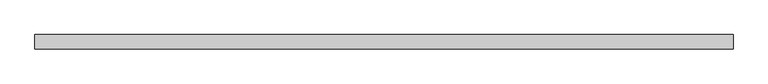
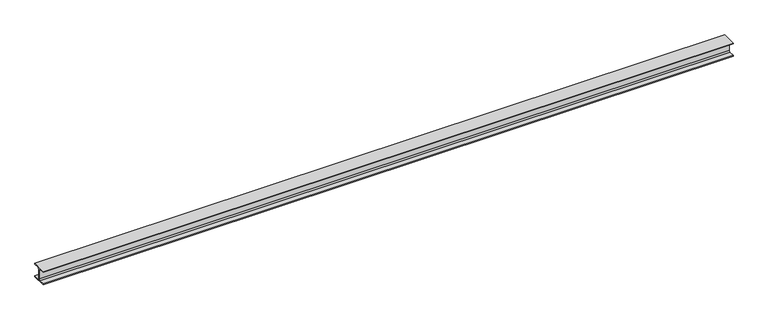
"""IFC4 building model written with IfcOpenShell, lengths in millimetres: beam geometry, NLRS_28_SF_LIB_stalen ligger HEB-AV-CWV-MMBS-SRP_gen_rsf : stalen ligger_gen__HEB 260."""

from ifc_helpers import new_model, si_unit, point, frame, frame_2d, origin, place, context, project, spatial, polyline, circle_curve, trimmed, segment, composite_curve, outline, extrude, source, transform, mapped, element, save


def beam_01d7d33a(model_context):
    return source(origin(), model_context, "Body", "SweptSolid", [
        extrude(outline(composite_curve([segment(polyline([(130.0, 112.5), (29.0, 112.5)]), True, "CONTINUOUS"), segment(trimmed(circle_curve(frame_2d((29.0, 88.5)), 24.0), [point((29.0, 112.5))], [point((5.0, 88.5))], True, "CARTESIAN"), True, "CONTINUOUS"), segment(polyline([(5.0, 88.5), (5.0, -88.5)]), True, "CONTINUOUS"), segment(trimmed(circle_curve(frame_2d((29.0, -88.5)), 24.0), [point((5.0, -88.5))], [point((29.0, -112.5))], True, "CARTESIAN"), True, "CONTINUOUS"), segment(polyline([(29.0, -112.5), (130.0, -112.5), (130.0, -130.0), (-130.0, -130.0), (-130.0, -112.5), (-29.0, -112.5)]), True, "CONTINUOUS"), segment(trimmed(circle_curve(frame_2d((-29.0, -88.5)), 24.0), [point((-29.0, -112.5))], [point((-5.0, -88.5))], True, "CARTESIAN"), True, "CONTINUOUS"), segment(polyline([(-5.0, -88.5), (-5.0, 88.5)]), True, "CONTINUOUS"), segment(trimmed(circle_curve(frame_2d((-29.0, 88.5)), 24.0), [point((-5.0, 88.5))], [point((-29.0, 112.5))], True, "CARTESIAN"), True, "CONTINUOUS"), segment(polyline([(-29.0, 112.5), (-130.0, 112.5), (-130.0, 130.0), (130.0, 130.0), (130.0, 112.5)]), True, "CONTINUOUS")], self_intersect=False)), frame((-6349.0, 0.0, 0.0), z_axis=(1.0, 0.0, 0.0), x_axis=(0.0, 1.0, 0.0)), (0.0, 0.0, 1.0), 12698.0),
    ])


if __name__ == "__main__":
    model = new_model("IFC4")
    model_context = context("Model", 3, world=origin())
    ifc_project = project(units=[si_unit("LENGTHUNIT", "METRE", prefix="MILLI")], contexts=[model_context])
    site = spatial("IfcSite", under=ifc_project)
    building = spatial("IfcBuilding", under=site)
    placement = place(None, origin())
    beam_shape = beam_01d7d33a(model_context)
    element("IfcBeam", 1, ObjectType="NLRS_28_SF_LIB_stalen ligger HEB-AV-CWV-MMBS-SRP_gen_rsf : stalen ligger_gen__HEB 260", at=placement, inside=building, context=model_context, shape_type="MappedRepresentation", body=[
        mapped(beam_shape, transform((0.0, 0.0, 0.0), x_axis=(1.0, 0.0, 0.0), y_axis=(0.0, 1.0, 0.0), z_axis=(0.0, 0.0, 1.0))),
    ])
    save(model, "model.ifc")

# Revit data of these elements
# Type "NLRS_28_SF_LIB_stalen ligger HEB-AV-CWV-MMBS-SRP_gen_rsf : stalen ligger_gen__HEB 260"
#   Type IfcGUID = "0zo1UjqZ91lRsfCKsOOa5a"
#   IfcExportAs = "IfcBeamType"
#   Type Comments = "HEB260"
#   Model = " "
#   Manufacturer = " "
#   Fire Rating = " "
#   Description = "stalen ligger HEB260"
#   Assembly Code = "28.11"
#   ra = 24 mm
#   vz = 130 mm
#   vy = 130 mm
#   vpz = 130 mm
#   vpy = 130 mm
#   NLRS_C_lengte [instance default] = 1500 mm
#   Length [instance default] = 1500 mm
#   bf = 260 mm
#   d = 260 mm
#   tf = 17.5 mm
#   tw = 10 mm
#   Structural Material = NLRS_h2_staal_gen_rsf
#   Keynote = ""
# Element 1 (IfcBeam, "NLRS_28_SF_LIB_stalen ligger HEB-AV-CWV-MMBS-SRP_gen_rsf : stalen ligger_gen__HEB 260")
#   NLRS_C_lengte = 12698 mm
#   Materials on its faces: "NLRS_h2_staal_gen_rsf"
# Materials
#   "NLRS_h2_staal_gen_rsf": class "H - Metaal", colour RGB 189 187 185, transparency 0, Keynote = "h2", Manufacturer = "Revit Standards Foundation", URL = "www.revitstandards.org", Description = "staal", Cost = 0
